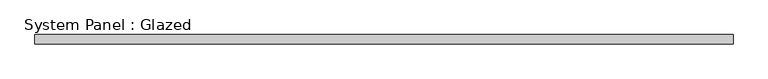
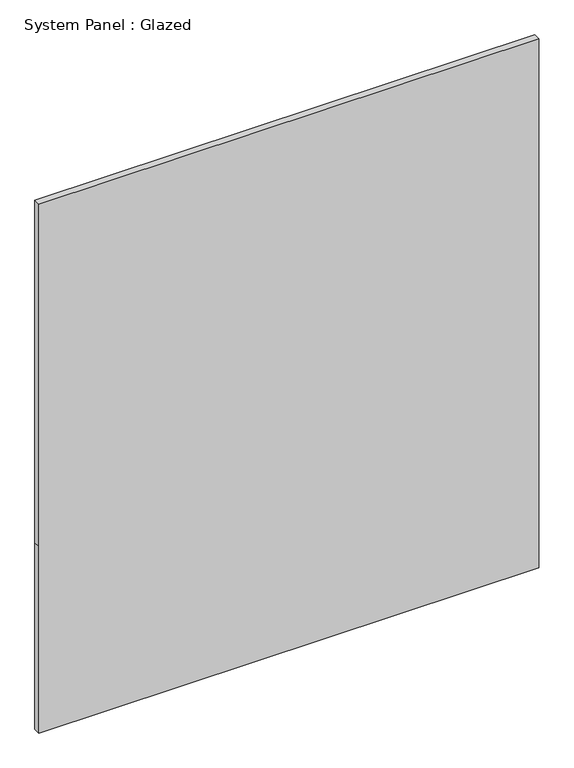
"""IFC4 building model written with IfcOpenShell, lengths in millimetres: plate geometry, System Panel : Glazed."""

from ifc_helpers import new_model, si_unit, frame, origin, place, context, project, spatial, polyline, outline, extrude, source, transform, mapped, element, save


def system_panel_glazed_635c0c9e(model_context):
    return source(origin(), model_context, "Body", "SweptSolid", [
        extrude(outline(polyline([(0.0, -949.9999998), (0.0, 949.9999998), (750.0, 949.9999998), (2125.0, 949.9999998), (2125.0, -949.9999998), (750.0, -949.9999998), (0.0, -949.9999998)])), frame((0.0, 24.5, 0.0), z_axis=(0.0, 1.0, 0.0), x_axis=(0.0, 0.0, 1.0)), (0.0, 0.0, 1.0), 25.0),
    ])


if __name__ == "__main__":
    model = new_model("IFC4")
    model_context = context("Model", 3, world=origin())
    ifc_project = project(units=[si_unit("LENGTHUNIT", "METRE", prefix="MILLI")], contexts=[model_context])
    site = spatial("IfcSite", under=ifc_project)
    building = spatial("IfcBuilding", under=site)
    placement = place(None, origin())
    system_panel_glazed_shape = system_panel_glazed_635c0c9e(model_context)
    element("IfcPlate", 1, ObjectType="System Panel : Glazed", at=placement, inside=building, context=model_context, shape_type="MappedRepresentation", body=[
        mapped(system_panel_glazed_shape, transform((0.0, 0.0, 0.0), x_axis=(1.0, 0.0, 0.0), y_axis=(0.0, 1.0, 0.0), z_axis=(0.0, 0.0, 1.0))),
    ])
    save(model, "model.ifc")

# Revit data of these elements
# Element 1 (IfcPlate, "System Panel : Glazed")
#   Materials on its faces: "Glass"
# Materials
#   "Glass": class "Glass", colour RGB 0 128 192, transparency 0.9
